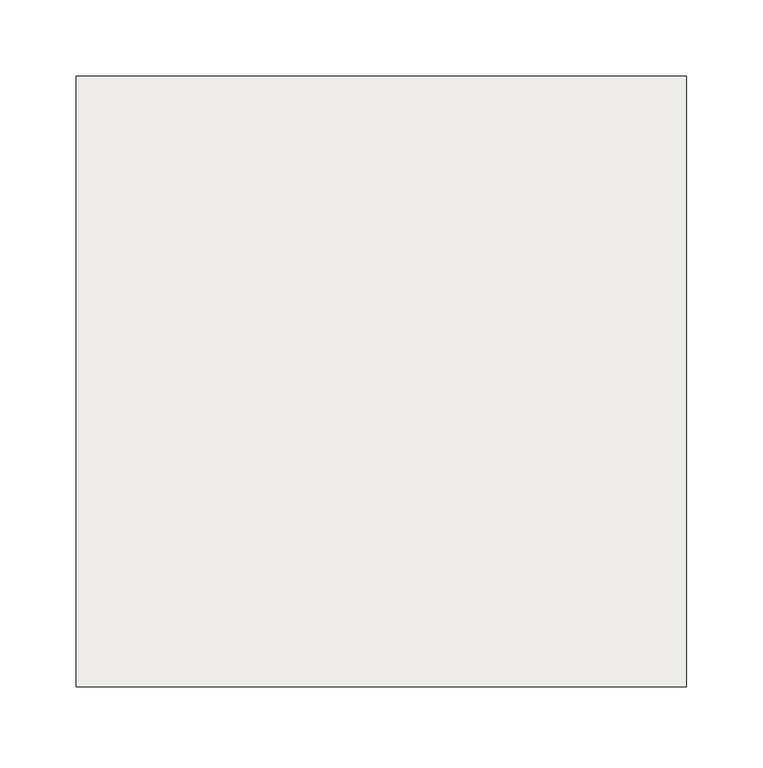
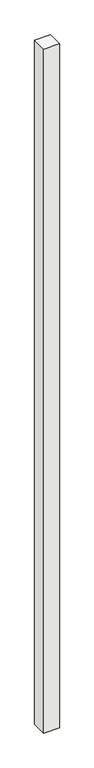
"""IFC4 building model written with IfcOpenShell, lengths in millimetres: slab geometry, NLRS_17_SFO_TLB_funderingspaal geheid beton prefab-AV-MMBPC_gen_rsf : heipaal beton prefab_gen__bxh 400x400."""

from ifc_helpers import new_model, si_unit, frame, origin, place, context, project, spatial, polyline, outline, extrude, source, transform, mapped, element, save


def slab_81e4ded3(model_context):
    return source(origin(), model_context, "Body", "SweptSolid", [
        extrude(outline(polyline([(200.0, -200.0), (-200.0, -200.0), (-200.0, 200.0), (200.0, 200.0), (200.0, -200.0)])), frame((0.0, 0.0, -20000.0), z_axis=(0.0, 0.0, 1.0), x_axis=(1.0, 0.0, 0.0)), (0.0, 0.0, 1.0), 18520.0),
    ])


if __name__ == "__main__":
    model = new_model("IFC4")
    model_context = context("Model", 3, world=origin())
    ifc_project = project(units=[si_unit("LENGTHUNIT", "METRE", prefix="MILLI")], contexts=[model_context])
    site = spatial("IfcSite", under=ifc_project)
    building = spatial("IfcBuilding", under=site)
    placement = place(None, origin())
    slab_shape = slab_81e4ded3(model_context)
    element("IfcSlab", 1, ObjectType="NLRS_17_SFO_TLB_funderingspaal geheid beton prefab-AV-MMBPC_gen_rsf : heipaal beton prefab_gen__bxh 400x400", at=placement, inside=building, context=model_context, shape_type="MappedRepresentation", body=[
        mapped(slab_shape, transform((0.0, 0.0, 0.0), x_axis=(1.0, 0.0, 0.0), y_axis=(0.0, 1.0, 0.0), z_axis=(0.0, 0.0, 1.0))),
    ])
    save(model, "model.ifc")

# Revit data of these elements
# Type "NLRS_17_SFO_TLB_funderingspaal geheid beton prefab-AV-MMBPC_gen_rsf : heipaal beton prefab_gen__bxh 400x400"
#   Export Type to IFC As = "IfcPile"
#   Type IfcGUID = "10$Kfo5uPCAOPJEOo5LE_W"
#   Type Comments = "prefab heipaal 400x400"
#   Model = " "
#   Manufacturer = " "
#   Description = "prefab heipaal 400x400"
#   Assembly Code = "17.21"
#   Width = 400 mm
#   Slanted Angle [instance default] = 0.00°
#   NLRS_S_draagvermogen_trek [instance default] = 0.00 kN
#   NLRS_S_draagvermogen_druk [instance default] = 0.00 kN
#   NLRS_C_lengte [instance default] = 1660 mm
#   NLRS_C_hoogte = 400 mm
#   NLRS_C_breedte = 400 mm
#   Height [instance default] = 1660 mm
#   Length [instance default] = 1660 mm
#   Angle [instance default] = 0.00°
#   Slanted [instance default] = 0
#   Structural Material = NLRS_f2_beton prefab_gen_rsf
#   Keynote = ""
# Element 1 (IfcSlab, "NLRS_17_SFO_TLB_funderingspaal geheid beton prefab-AV-MMBPC_gen_rsf : heipaal beton prefab_gen__bxh 400x400")
#   NLRS_C_lengte = 18520 mm
#   Height = 18520 mm
#   Length = 18520 mm
#   Materials on its faces: "NLRS_f2_beton prefab_gen_rsf"
# Materials
#   "NLRS_f2_beton prefab_gen_rsf": class "F - Niet gebakken kunststeen", colour RGB 129 133 118, transparency 0, Keynote = "f2", Manufacturer = "Revit Standards Foundation", URL = "www.revitstandards.org", Description = "beton prefab", Cost = 0
